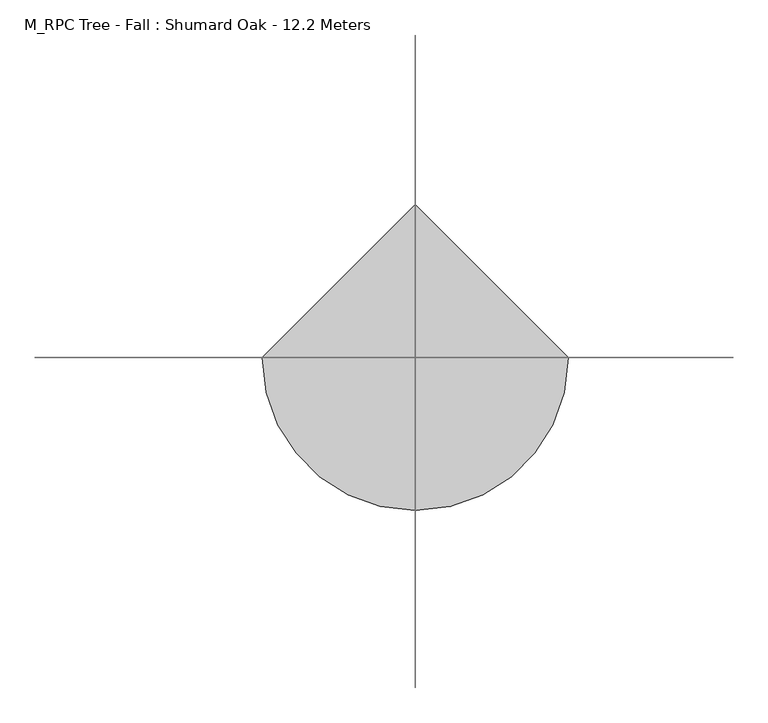
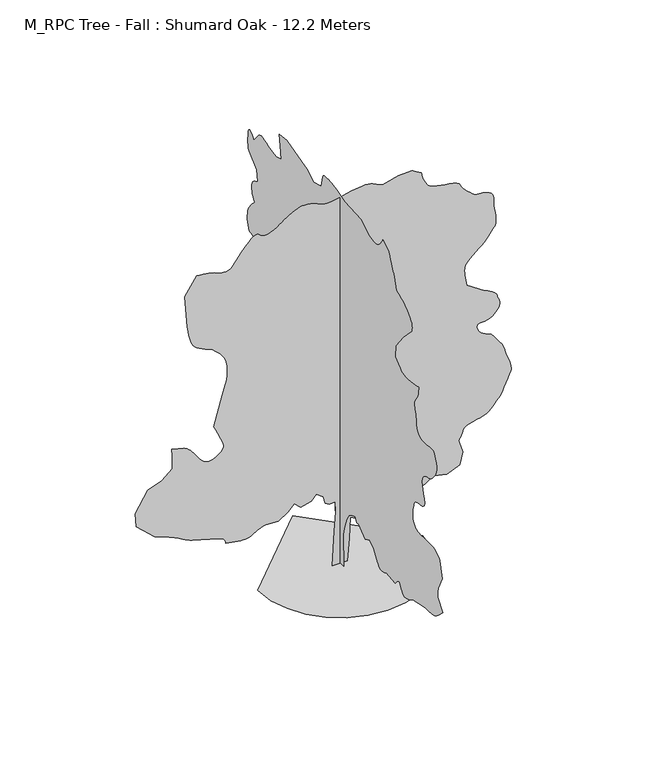
"""IFC4 building model written with IfcOpenShell, lengths in millimetres: geographic element geometry, M_RPC Tree - Fall : Shumard Oak - 12.2 Meters."""

from ifc_helpers import new_model, si_unit, origin, place, context, project, spatial, triangles, source, transform, mapped, element, save


def m_rpc_tree_fall_shumard_oak_12_2_meters_a262d815(model_context):
    return source(origin(), model_context, "Body", "Tessellation", [
        triangles([(-0.0022625, 219.6430976, 0.0114771), (-0.0022625, -202.2794772, 0.0114771), (-0.0022625, -165.5900743, 1045.6450413), (-0.0022625, -238.9678628, 1357.501878), (-0.0022625, -349.0363624, 1651.0131775), (-0.0022625, -477.4462206, 1852.8008606), (-0.0022625, -624.2017977, 1944.5243317), (-0.0022625, -807.646269, 2017.9021202), (-0.0022625, -881.0241302, 1852.8008606), (-0.0022625, -1009.4364956, 1889.4897549), (-0.0022625, -1156.1920727, 1742.7340324), (-0.0022625, -1357.9797558, 1614.3242832), (-0.0022625, -1596.4563332, 1724.390966), (-0.0022625, -1816.5896988, 1577.6353889), (-0.0022625, -1963.347892, 1320.8129837), (-0.0022625, -1998.8599686, 1270.1093925), (-0.0022625, -2035.172723, 1221.8152473), (-0.0022625, -2073.0917747, 1178.3350525), (-0.0022625, -2113.4178017, 1142.073167), (-0.0022625, -2156.9513363, 1115.4391096), (-0.0022625, -2204.4982887, 1100.8397827), (-0.0022625, -2256.8565754, 1100.6771473), (-0.0022625, -2307.0772018, 1109.6110497), (-0.0022625, -2348.6333862, 1120.4664917), (-0.0022625, -2382.9686451, 1132.928231), (-0.0022625, -2411.5294018, 1146.673613), (-0.0022625, -2435.7565567, 1161.3821629), (-0.0022625, -2457.0962425, 1176.7312986), (-0.0022625, -2476.9897957, 1192.4006184), (-0.0022625, -2953.9455666, 1137.368585), (-0.0022625, -3000.966243, 1191.6508095), (-0.0022625, -3046.9957008, 1241.4419563), (-0.0022625, -3091.1191704, 1282.250948), (-0.0022625, -3132.3701408, 1309.5814018), (-0.0022625, -3169.7582657, 1318.9398422), (-0.0022625, -3202.3167435, 1305.8375896), (-0.0022625, -3229.1060966, 1265.7784069), (-0.0022625, -3256.0221863, 1208.176763), (-0.0022625, -3289.3434082, 1148.6509632), (-0.0022625, -3328.7392593, 1092.0151033), (-0.0022625, -3373.9553947, 1043.0779741), (-0.0022625, -3424.5851532, 1006.655924), (-0.0022625, -3480.3747711, 987.5629761), (-0.0022625, -3540.9678749, 990.6103918), (-0.0022625, -3601.7135857, 1008.4757984), (-0.0022625, -3658.6214493, 1030.1891533), (-0.0022625, -3712.3268921, 1055.1127047), (-0.0022625, -3763.4650497, 1082.6007797), (-0.0022625, -3812.6716393, 1112.0180248), (-0.0022625, -3860.5820869, 1142.7162237), (-0.0022625, -3907.8568176, 1174.0574793), (-0.0022625, -4568.2572052, 1302.4673012), (-0.0022625, -4650.6324097, 1302.6274658), (-0.0022625, -4731.8637886, 1303.7507984), (-0.0022625, -4810.8586761, 1306.8009029), (-0.0022625, -4886.4732468, 1312.7355698), (-0.0022625, -4957.6142532, 1322.5236351), (-0.0022625, -5023.1381607, 1337.1228893), (-0.0022625, -5081.9014343, 1357.501878), (-0.0022625, -5138.5299545, 1386.9699921), (-0.0022625, -5198.0553909, 1427.0265587), (-0.0022625, -5259.9957962, 1475.9103481), (-0.0022625, -5323.8680603, 1531.8524277), (-0.0022625, -5389.1634933, 1593.0911316), (-0.0022625, -5455.4245651, 1657.8578178), (-0.0022625, -5522.1681656, 1724.390966), (-0.0022625, -5265.3588409, 2017.9021202), (-0.0022625, -5257.7087265, 2072.8807411), (-0.0022625, -5251.3288834, 2127.5393234), (-0.0022625, -5247.5419052, 2181.5572472), (-0.0022625, -5247.5924835, 2234.6118576), (-0.0022625, -5252.7776321, 2286.3829708), (-0.0022625, -5264.3932022, 2336.5504028), (-0.0022625, -5283.6844666, 2384.7910629), (-0.0022625, -5485.4924973, 2806.7071701), (-0.0022625, -5357.0619644, 3320.3516899), (-0.0022625, -5347.0224609, 3334.5342545), (-0.0022625, -5317.0562668, 3370.8544212), (-0.0022625, -5267.544754, 3419.9848526), (-0.0022625, -5198.7675568, 3472.673497), (-0.0022625, -5111.054306, 3519.5671463), (-0.0022625, -5004.7369583, 3551.3887505), (-0.0022625, -4880.1189835, 3558.8359703), (-0.0022625, -4741.2681564, 3553.0662643), (-0.0022625, -4598.2742683, 3550.8041931), (-0.0022625, -4460.38908, 3551.1346962), (-0.0022625, -4336.9405106, 3553.0662643), (-0.0022625, -4237.2564789, 3555.6332588), (-0.0022625, -4170.614035, 3557.8700409), (-0.0022625, -4146.341098, 3558.8359703), (-0.0022625, -4132.1076645, 3568.5196815), (-0.0022625, -4095.4317055, 3595.8424324), (-0.0022625, -4045.2591866, 3638.2628082), (-0.0022625, -3990.588105, 3693.1882347), (-0.0022625, -3940.4411659, 3758.0514267), (-0.0022625, -3903.7393364, 3830.3106789), (-0.0022625, -3889.5061935, 3907.3739983), (-0.0022625, -3892.2002151, 3984.3864487), (-0.0022625, -3899.6727242, 4058.5266907), (-0.0022625, -3911.1609764, 4130.2522545), (-0.0022625, -3925.8772293, 4200.0465408), (-0.0022625, -3943.0081604, 4268.3917877), (-0.0022625, -3961.7148674, 4335.7711052), (-0.0022625, -3981.2346062, 4402.667894), (-0.0022625, -3997.2725807, 4422.2640816), (-0.0022625, -4015.2421234, 4441.35187), (-0.0022625, -4037.0750931, 4459.4740196), (-0.0022625, -4064.677478, 4476.1727097), (-0.0022625, -4099.9558479, 4490.9142517), (-0.0022625, -4144.8923492, 4503.2922752), (-0.0022625, -4201.3679718, 4512.7472214), (-0.0022625, -4269.6626404, 4518.5166367), (-0.0022625, -4343.4215103, 4525.252272), (-0.0022625, -4414.6136765, 4540.6545296), (-0.0022625, -4475.2067802, 4572.4255554), (-0.0022625, -4517.1952057, 4628.2657516), (-0.0022625, -4532.5213051, 4715.8769737), (-0.0022625, -4513.2300407, 4842.9346252), (-0.0022625, -4473.7071625, 4986.5892288), (-0.0022625, -4437.3869957, 5118.3747894), (-0.0022625, -4409.7337418, 5237.654718), (-0.0022625, -4396.2118927, 5343.7435913), (-0.0022625, -4402.2612328, 5436.0571426), (-0.0022625, -4433.3200928, 5513.9332031), (-0.0022625, -4494.8794167, 5576.7125107), (-0.0022625, -4570.3413803, 5620.6830826), (-0.0022625, -4640.3641411, 5647.6500412), (-0.0022625, -4706.1929718, 5665.2896622), (-0.0022625, -4769.1501755, 5681.3276367), (-0.0022625, -4830.4804436, 5703.465239), (-0.0022625, -4891.5054977, 5739.4299042), (-0.0022625, -4953.4970627, 5796.846167), (-0.0022625, -5016.6571609, 5869.9184509), (-0.0022625, -5076.9197617, 5947.7950928), (-0.0022625, -5129.1764557, 6030.7807251), (-0.0022625, -5168.2670929, 6119.2555573), (-0.0022625, -5189.0838455, 6213.4753876), (-0.0022625, -5186.4654007, 6313.8198441), (-0.0022625, -5155.2795135, 6420.5697235), (-0.0022625, -5117.6376251, 6521.5501877), (-0.0022625, -5092.1699936, 6603.8998123), (-0.0022625, -5068.6342209, 6667.0093323), (-0.0022625, -5036.7617477, 6710.2177414), (-0.0022625, -4986.2845963, 6732.9146118), (-0.0022625, -4906.908046, 6734.4145203), (-0.0022625, -4788.3905708, 6714.0808777), (-0.0022625, -4647.7857811, 6691.613063), (-0.0022625, -4512.6454834, 6687.1139191), (-0.0022625, -4388.3835915, 6700.6101883), (-0.0022625, -4280.5154663, 6732.0507111), (-0.0022625, -4194.4803108, 6781.4604858), (-0.0022625, -4135.6914574, 6848.8656738), (-0.0022625, -4109.6395592, 6934.214534), (-0.0022625, -4100.7183014, 7025.3583893), (-0.0022625, -4089.8654755, 7110.7072495), (-0.0022625, -4077.385714, 7191.2529144), (-0.0022625, -4063.6609703, 7267.9348618), (-0.0022625, -4048.9447174, 7341.7448914), (-0.0022625, -4033.5930382, 7413.6230621), (-0.0022625, -4017.9364357, 7484.5350128), (-0.0022625, -4002.6864944, 7535.6737518), (-0.0022625, -3990.3337601, 7586.9642258), (-0.0022625, -3983.7510223, 7638.5854935), (-0.0022625, -3985.8351974, 7690.6642914), (-0.0022625, -3999.483783, 7743.4035141), (-0.0022625, -4027.5436981, 7796.9310608), (-0.0022625, -4072.9633095, 7851.4242462), (-0.0022625, -4121.5091835, 7918.2951645), (-0.0022625, -4158.2107224, 8002.1446976), (-0.0022625, -4184.6184128, 8093.0600784), (-0.0022625, -4202.3847702, 8181.1029602), (-0.0022625, -4213.0852798, 8256.2855804), (-0.0022625, -4218.3210068, 8308.7201706), (-0.0022625, -4219.7188866, 8328.392807), (-0.0022625, -4192.65019, 8322.3431763), (-0.0022625, -4120.0348549, 8306.9917877), (-0.0022625, -4014.6575661, 8286.5058289), (-0.0022625, -3889.4044556, 8265.0798111), (-0.0022625, -3757.0854973, 8246.830925), (-0.0022625, -3630.5615341, 8235.9775177), (-0.0022625, -3522.6172508, 8236.6641037), (-0.0022625, -3431.498394, 8252.5491806), (-0.0022625, -3346.123954, 8282.871167), (-0.0022625, -3265.5788704, 8325.2406738), (-0.0022625, -3188.8969231, 8377.2177338), (-0.0022625, -3115.0868935, 8436.4385376), (-0.0022625, -3043.2087227, 8500.4375381), (-0.0022625, -2972.2964813, 8566.876506), (-0.0022625, -2990.6471054, 8952.1163635), (-0.0022625, -3394.2122978, 9465.761174), (-0.0022625, -3852.8299438, 9942.7035736), (-0.0022625, -3859.9975296, 10001.8488007), (-0.0022625, -3862.9964745, 10062.1369812), (-0.0022625, -3857.6337204, 10124.6622345), (-0.0022625, -3839.7659157, 10190.5419342), (-0.0022625, -3805.2247101, 10260.9201965), (-0.0022625, -3749.8164642, 10336.9155579), (-0.0022625, -3669.3728279, 10419.6721344), (-0.0022625, -3575.0262611, 10499.1754211), (-0.0022625, -3480.7049835, 10566.1992371), (-0.0022625, -3386.3587074, 10622.777179), (-0.0022625, -3292.0121407, 10671.0172577), (-0.0022625, -3197.6655739, 10713.0053925), (-0.0022625, -3103.3190071, 10750.825177), (-0.0022625, -3008.9724403, 10786.535788), (-0.0022625, -2981.4465042, 10880.6288818), (-0.0022625, -2953.7423813, 10973.0941681), (-0.0022625, -2925.7077553, 11062.3573242), (-0.0022625, -2897.1903099, 11146.8172852), (-0.0022625, -2868.0627274, 11224.8462433), (-0.0022625, -2838.0965332, 11294.8431335), (-0.0022625, -2807.1899895, 11355.2324707), (-0.0022625, -2772.9028381, 11421.0621735), (-0.0022625, -2735.1083427, 11502.2932617), (-0.0022625, -2696.9580551, 11589.6507202), (-0.0022625, -2661.7305542, 11673.779306), (-0.0022625, -2632.5776825, 11745.3784241), (-0.0022625, -2612.7274406, 11795.1695709), (-0.0022625, -2605.4075386, 11813.8509888), (-0.0022625, -2293.5479404, 11997.2828156), (-0.0022625, -2277.555748, 11965.6638153), (-0.0022625, -2259.9598743, 11933.1053375), (-0.0022625, -2239.1538769, 11898.6155823), (-0.0022625, -2213.5363998, 11861.2271667), (-0.0022625, -2181.5012913, 11819.9761963), (-0.0022625, -2141.4421085, 11773.9464478), (-0.0022625, -2091.7577866, 11722.1217041), (-0.0022625, -2031.9117302, 11677.2360718), (-0.0022625, -1963.4012318, 11650.6760651), (-0.0022625, -1887.6698078, 11639.3151306), (-0.0022625, -1806.1612656, 11640.1790314), (-0.0022625, -1720.3217377, 11650.1935364), (-0.0022625, -1631.594886, 11666.2820892), (-0.0022625, -1541.4242271, 11685.4204559), (-0.0022625, -1137.8463902, 11960.5804047), (-0.0022625, -257.3128368, 12015.6328583), (-0.0022625, -143.5556361, 12046.9216461), (-0.0022625, -31.2426242, 12077.2430511), (-0.0022625, 78.1820465, 12105.6331787), (-0.0022625, 183.2749686, 12131.1513885), (-0.0022625, 282.5921986, 12152.8070435), (-0.0022625, 374.6893387, 12169.6583405), (-0.0022625, 458.1194206, 12180.7390594), (-0.0022625, 540.3752283, 12189.1780792), (-0.0022625, 626.4842165, 12196.675296), (-0.0022625, 711.3070913, 12199.9797455), (-0.0022625, 789.7123346, 12195.9137146), (-0.0022625, 856.5631233, 12181.2739105), (-0.0022625, 906.7304827, 12152.8070435), (-0.0022625, 935.0776623, 12107.3365631), (-0.0022625, 1026.7985899, 11740.4729095), (-0.0022625, 1430.3764996, 11630.3935822), (-0.0022625, 1797.2654423, 11850.5266571), (-0.0022625, 2255.8780014, 11960.5804047), (-0.0022625, 2861.2512245, 12144.0378113), (-0.0022625, 3264.8164169, 12089.0109375), (-0.0022625, 3228.1401672, 11740.4729095), (-0.0022625, 3154.7623787, 11336.882428), (-0.0022625, 3448.2735329, 11245.1531433), (-0.0022625, 3741.784687, 11300.1811798), (-0.0022625, 3855.2699112, 11342.8297394), (-0.0022625, 3965.7050308, 11381.7424805), (-0.0022625, 4070.0405228, 11413.310321), (-0.0022625, 4165.2509903, 11433.7962799), (-0.0022625, 4248.2619118, 11439.5145355), (-0.0022625, 4316.0226013, 11426.7804291), (-0.0022625, 4365.4832451, 11391.9093018), (-0.0022625, 4640.6437752, 11061.7213165), (-0.0022625, 4703.1684471, 11134.820343), (-0.0022625, 4763.4566277, 11198.46297), (-0.0022625, 4819.2209564, 11243.1707062), (-0.0022625, 4868.274939, 11259.4883148), (-0.0022625, 4908.3317963, 11237.9349792), (-0.0022625, 4937.1538742, 11169.0566254), (-0.0022625, 4952.5058441, 11043.3712738), (-0.0022625, 4957.156723, 10903.7832825), (-0.0022625, 4956.038768, 10795.9654449), (-0.0022625, 4950.1164551, 10714.6064575), (-0.0022625, 4940.305426, 10654.4461761), (-0.0022625, 4927.6480591, 10610.169809), (-0.0022625, 4913.0338348, 10576.467215), (-0.0022625, 4897.478389, 10548.0770874), (-0.0022625, 4475.5625725, 10199.5134796), (-0.0022625, 4438.8610336, 9814.2997833), (-0.0022625, 4497.5481491, 9790.3826385), (-0.0022625, 4554.4304329, 9764.5586334), (-0.0022625, 4607.8053726, 9734.8726547), (-0.0022625, 4655.8937164, 9699.416098), (-0.0022625, 4696.9159218, 9656.2588486), (-0.0022625, 4729.118898, 9603.4684662), (-0.0022625, 4750.7231026, 9539.1136734), (-0.0022625, 4758.958065, 9468.3790375), (-0.0022625, 4753.7223381, 9397.6194031), (-0.0022625, 4737.2521225, 9326.8591873), (-0.0022625, 4711.7847816, 9256.0995529), (-0.0022625, 4679.5818054, 9185.3393372), (-0.0022625, 4642.9058464, 9114.5797028), (-0.0022625, 4603.9675255, 9043.819487), (-0.0022625, 4662.6799301, 8984.827739), (-0.0022625, 4719.9688751, 8925.6830933), (-0.0022625, 4774.3606133, 8866.2082352), (-0.0022625, 4824.4313942, 8806.250267), (-0.0022625, 4868.7068893, 8745.6574539), (-0.0022625, 4905.7645111, 8684.2763168), (-0.0022625, 4934.1546387, 8621.9039612), (-0.0022625, 4954.5388596, 8561.1582504), (-0.0022625, 4969.1536652, 8504.2500961), (-0.0022625, 4978.9391144, 8450.5446533), (-0.0022625, 4984.8608459, 8399.4064957), (-0.0022625, 4987.9112411, 8350.2001968), (-0.0022625, 4989.0291962, 8302.2897491), (-0.0022625, 4989.2070923, 8255.0147278), (-0.0022625, 4879.1277649, 7943.1529495), (-0.0022625, 4828.0657654, 7934.9685654), (-0.0022625, 4777.130793, 7924.8784836), (-0.0022625, 4726.5519035, 7910.8991043), (-0.0022625, 4676.4302536, 7891.1758896), (-0.0022625, 4626.9696098, 7863.7258209), (-0.0022625, 4578.2967087, 7826.6681992), (-0.0022625, 4530.5897369, 7778.046167), (-0.0022625, 4487.1525627, 7720.3508514), (-0.0022625, 4450.476313, 7657.8255981), (-0.0022625, 4419.3918732, 7591.3104721), (-0.0022625, 4392.8059959, 7521.5670547), (-0.0022625, 4369.6007263, 7449.4092499), (-0.0022625, 4348.6319481, 7375.6503799), (-0.0022625, 4328.8069954, 7301.103186), (-0.0022625, 4285.8529312, 7242.111438), (-0.0022625, 4244.6781189, 7182.9667923), (-0.0022625, 4207.0106506, 7123.4919342), (-0.0022625, 4174.6553581, 7063.5339661), (-0.0022625, 4149.3656227, 7002.941153), (-0.0022625, 4132.8956978, 6941.534436), (-0.0022625, 4126.9989647, 6879.1876602), (-0.0022625, 4145.3498795, 6383.8684753), (-0.0022625, 4188.3039436, 6379.5472275), (-0.0022625, 4229.478756, 6372.8121735), (-0.0022625, 4267.1462242, 6361.2477631), (-0.0022625, 4299.5018074, 6342.4901871), (-0.0022625, 4324.7912521, 6314.0744797), (-0.0022625, 4341.2611771, 6273.6618301), (-0.0022625, 4347.1323303, 6218.7872726), (-0.0022625, 4345.5312653, 6155.3475403), (-0.0022625, 4341.0579918, 6090.9671677), (-0.0022625, 4334.1444603, 6025.7734726), (-0.0022625, 4325.3249405, 5959.9187714), (-0.0022625, 4315.0566719, 5893.6071213), (-0.0022625, 4303.8224739, 5826.9646774), (-0.0022625, 4292.1054565, 5760.1699173), (-0.0022625, 4273.7545418, 5393.2806839), (-0.0022625, 4622.3181496, 5411.631308), (-0.0022625, 5007.5327179, 5485.0093872), (-0.0022625, 5089.5265503, 5457.2541046), (-0.0022625, 5168.1403564, 5428.0506546), (-0.0022625, 5240.0441071, 5395.949707), (-0.0022625, 5301.8060349, 5359.5275116), (-0.0022625, 5350.0978546, 5317.3359009), (-0.0022625, 5381.5383774, 5267.9261261), (-0.0022625, 5392.7725754, 5209.8232773), (-0.0022625, 5389.5698639, 5136.2423035), (-0.0022625, 5380.5721573, 5043.3956451), (-0.0022625, 5366.7968353, 4934.5104309), (-0.0022625, 5349.1322159, 4812.790535), (-0.0022625, 5328.5956787, 4681.4372154), (-0.0022625, 5306.1272827, 4543.6537651), (-0.0022625, 5282.7182465, 4402.667894), (-0.0022625, 5117.6120453, 3962.400872), (-0.0022625, 5027.4338287, 3911.8219826), (-0.0022625, 4938.704361, 3864.2673271), (-0.0022625, 4852.8723907, 3822.8128807), (-0.0022625, 4771.3613777, 3790.5084572), (-0.0022625, 4695.6453598, 3770.4038704), (-0.0022625, 4627.1219261, 3765.5492249), (-0.0022625, 4567.2659866, 3778.9693359), (-0.0022625, 4053.6211761, 3999.1027016), (-0.0022625, 3539.9766563, 3833.9962097), (-0.0022625, 3173.0877136, 3577.1865944), (-0.0022625, 2806.1987709, 3026.8405357), (-0.0022625, 2770.6916359, 2972.1438744), (-0.0022625, 2734.3967583, 2919.353492), (-0.0022625, 2696.4752357, 2870.4012474), (-0.0022625, 2656.139035, 2827.2437073), (-0.0022625, 2612.6004135, 2791.7874413), (-0.0022625, 2565.0713379, 2765.9643082), (-0.0022625, 2512.700116, 2751.6800056), (-0.0022625, 2460.4463287, 2746.9270981), (-0.0022625, 2411.4048454, 2747.2828903), (-0.0022625, 2362.0407074, 2751.1971863), (-0.0022625, 2308.8259323, 2757.0174706), (-0.0022625, 2248.2300671, 2763.1682579), (-0.0022625, 2176.7229492, 2768.0484833), (-0.0022625, 2090.7765965, 2770.0309204), (-0.0022625, 1998.5727768, 2763.0668106), (-0.0022625, 1910.2194489, 2743.5976501), (-0.0022625, 1825.0763901, 2713.7076141), (-0.0022625, 1742.5003258, 2675.4555885), (-0.0022625, 1661.8482719, 2630.9766174), (-0.0022625, 1582.4797153, 2582.3037163), (-0.0022625, 1503.7542881, 2531.54664), (-0.0022625, 1393.6876053, 2219.6898033), (-0.0022625, 1081.8332394, 1871.1465431), (-0.0022625, 1038.7799807, 1824.5095642), (-0.0022625, 988.9862904, 1778.8358986), (-0.0022625, 933.5780445, 1733.9627655), (-0.0022625, 873.678721, 1689.7327618), (-0.0022625, 810.4091091, 1645.9857227), (-0.0022625, 744.8926867, 1602.5563969), (-0.0022625, 678.2553297, 1559.2895611), (-0.0022625, 568.1886469, 1944.5243317), (-0.0022625, 384.7416321, 2201.3465916), (-0.0022625, 311.3663507, 2036.245332), (-0.0022625, 256.3317375, 1779.4229267), (-0.0022625, 237.9877991, 1320.8129837), (-0.0022625, 201.2983961, 678.7560259), (227.2985896, 0.0005818, 0.0290512), (-249.6563274, 0.0005818, 0.0290512), (-176.2792837, 0.0005163, 1100.6948788), (-139.5901351, 0.0004777, 1742.7519093), (-157.9345822, 0.0004581, 2072.9519577), (-341.3808703, 0.0004592, 2054.608746), (-469.7907286, 0.000455, 2127.9865345), (-524.8227983, 0.0004406, 2366.4631119), (-744.9587437, 0.0004319, 2513.218689), (-891.7143208, 0.0004417, 2348.1174294), (-1221.9118984, 0.0004473, 2256.3964291), (-1423.7020523, 0.0004364, 2439.8409004), (-1625.4897354, 0.0004483, 2238.0507465), (-1919.0008896, 0.0004592, 2054.608746), (-2359.270237, 0.0004581, 2072.9519577), (-2579.4062187, 0.0004637, 1981.2284866), (-2626.6812401, 0.0004658, 1946.0925499), (-2674.5913971, 0.0004679, 1912.3976589), (-2723.7979866, 0.0004697, 1881.5927078), (-2774.9361443, 0.0004711, 1855.1187424), (-2828.6415871, 0.0004725, 1834.4220406), (-2885.5241615, 0.0004732, 1820.9436481), (-2946.2951614, 0.0004735, 1816.1296978), (-3014.004982, 0.0004735, 1818.2698288), (-3090.3820061, 0.0004732, 1824.2579807), (-3173.9771942, 0.0004725, 1833.4587273), (-3263.3420883, 0.0004718, 1845.2241428), (-3357.0279396, 0.0004711, 1858.9160397), (-3453.6362869, 0.00047, 1873.8915791), (-3551.6683846, 0.0004693, 1889.5074863), (-3556.192527, 0.0004669, 1928.7100353), (-3564.4527786, 0.0004644, 1967.2696003), (-3580.0588028, 0.0004623, 2004.5482841), (-3606.7461273, 0.0004602, 2039.9001961), (-3648.2005737, 0.0004581, 2072.6851135), (-3708.0823837, 0.0004564, 2102.2599072), (-3790.1270851, 0.000455, 2127.9865345), (-4597.2827591, 0.0004406, 2366.4631119), (-4663.1883293, 0.0004396, 2387.3759342), (-4733.5668823, 0.0004378, 2416.9507278), (-4806.1822174, 0.0004357, 2452.6229691), (-4878.822551, 0.0004333, 2491.825518), (-4949.2013947, 0.0004308, 2531.9913803), (-5015.1066742, 0.0004287, 2570.5611191), (-5074.2513199, 0.0004266, 2604.9500084), (-5137.8433685, 0.0004245, 2637.9915962), (-5216.8385468, 0.0004224, 2673.9306816), (-5308.668988, 0.00042, 2712.2844452), (-5410.7674072, 0.0004179, 2752.5441971), (-5520.5671005, 0.0004154, 2794.2782776), (-5635.5013641, 0.0004126, 2836.9527077), (-5753.0023315, 0.0004101, 2880.1102478), (-6321.6740158, 0.0003783, 3412.1056824), (-6358.3502655, 0.000352, 3852.3724136), (-5973.1354065, 0.0003149, 4476.0709717), (-5532.8686752, 0.0003051, 4641.1774635), (-5202.6562729, 0.0002886, 4916.3377029), (-5202.6562729, 0.0002637, 5338.2538101), (-5221.006897, 0.0002504, 5558.3868851), (-4835.7670395, 0.000256, 5466.6837616), (-4792.4063141, 0.0002578, 5438.7000046), (-4748.2066864, 0.0002595, 5407.9972275), (-4702.4315735, 0.0002616, 5371.8546661), (-4654.2414917, 0.0002641, 5327.5027222), (-4602.8489891, 0.0002676, 5272.2723724), (-4547.4407433, 0.0002718, 5203.3928558), (-4487.2290115, 0.0002767, 5118.1201538), (-4426.2036667, 0.000282, 5028.5523651), (-4367.4148132, 0.0002869, 4949.5571869), (-4308.6515396, 0.0002907, 4882.7624268), (-4247.6264854, 0.0002939, 4829.7432793), (-4182.1022873, 0.0002963, 4792.1522598), (-4109.8427444, 0.0002974, 4771.564563), (-4028.6113655, 0.0002974, 4769.5821259), (-3939.7801598, 0.0002963, 4789.9154778), (-3850.3138184, 0.0002939, 4831.0902901), (-3766.2863892, 0.0002904, 4887.032515), (-3693.823661, 0.0002865, 4951.641362), (-3638.9999725, 0.0002827, 5018.8174942), (-3607.915242, 0.0002788, 5082.4607025), (-3606.6952583, 0.0002756, 5136.4713593), (-3628.2994629, 0.0002721, 5194.8788406), (-3660.5024391, 0.0002676, 5273.4920654), (-3701.5246445, 0.0002616, 5368.9571686), (-3749.5876991, 0.0002553, 5477.9179596), (-3802.9626389, 0.0002483, 5596.9694138), (-3859.8702118, 0.0002406, 5722.7565033), (-3918.5573273, 0.0002329, 5851.8980392), (-3661.7224228, 0.0001772, 6787.4845367), (-3626.5966599, 0.0001709, 6893.3699341), (-3592.8940659, 0.0001646, 6997.8321625), (-3562.0892601, 0.0001587, 7099.3968933), (-3535.6051208, 0.0001527, 7196.6159592), (-3514.9159767, 0.0001475, 7288.064447), (-3501.4449966, 0.0001422, 7372.2953522), (-3496.6159309, 0.000138, 7447.884343), (-3497.8612038, 0.0001334, 7521.6182144), (-3501.9789757, 0.0001289, 7599.875647), (-3509.6293808, 0.000124, 7680.3701523), (-3521.4478455, 0.0001191, 7760.8646576), (-3538.0703773, 0.0001145, 7839.0970917), (-3560.1574013, 0.00011, 7912.8559616), (-3588.3446342, 0.0001061, 7979.8541977), (-3624.613932, 0.0001023, 8042.2265533), (-3669.5251442, 9.88e-05, 8103.6332703), (-3721.6801003, 9.53e-05, 8164.2266647), (-3779.6047623, 9.14e-05, 8224.1846329), (-3841.8500908, 8.79e-05, 8283.6339111), (-3906.9926262, 8.44e-05, 8342.8035553), (-3973.584201, 8.09e-05, 8401.7958847), (-4079.2667038, 7.85e-05, 8445.1054504), (-4182.2040253, 7.57e-05, 8488.8987076), (-4279.7021439, 7.32e-05, 8533.6826019), (-4369.0414581, 7.04e-05, 8579.8902466), (-4447.4264992, 6.76e-05, 8628.0291687), (-4512.213533, 6.44e-05, 8678.5574799), (-4560.6068001, 6.13e-05, 8731.9832886), (-4598.6809296, 5.71e-05, 8803.226033), (-4633.8828506, 5.15e-05, 8899.8090912), (-4665.5265587, 4.48e-05, 9011.1592712), (-4693.0272057, 3.78e-05, 9126.6778015), (-4715.6990776, 3.12e-05, 9235.7914902), (-4732.931456, 2.59e-05, 9327.8759857), (-4744.0383362, 2.21e-05, 9392.3830948), (-4817.4161247, -3.92e-05, 10419.6721344), (-4450.527182, -7.32e-05, 10988.3444), (-4352.4953751, -7.25e-05, 10976.4241974), (-4255.9123169, -7.18e-05, 10963.6900909), (-4162.2011765, -7.08e-05, 10949.3549194), (-4072.8362823, -6.97e-05, 10932.6303589), (-3989.2410942, -6.86e-05, 10912.6792511), (-3912.8893593, -6.72e-05, 10888.7109467), (-3845.1795387, -6.55e-05, 10859.939447), (-3776.3258926, -6.37e-05, 10832.1330048), (-3698.8306229, -6.27e-05, 10812.6644257), (-3617.497506, -6.2e-05, 10803.1336121), (-3537.1047386, -6.23e-05, 10805.1660461), (-3462.5069664, -6.3e-05, 10820.3651184), (-3398.482386, -6.48e-05, 10850.3063141), (-3349.8603539, -6.76e-05, 10896.6406952), (-3056.3491997, -9.07e-05, 11281.8555542), (-2977.9641586, -9.6e-05, 11371.601239), (-2900.8246811, -0.0001012, 11457.3320526), (-2826.2777779, -0.0001058, 11535.0552155), (-2755.5687218, -0.0001096, 11600.7326019), (-2689.9939453, -0.0001128, 11650.3714325), (-2630.8492996, -0.0001145, 11679.9300934), (-2579.4062187, -0.0001149, 11685.4460358), (-2538.0075829, -0.0001138, 11671.6445526), (-2504.3128372, -0.0001124, 11649.1761566), (-2472.5444275, -0.000111, 11622.8696228), (-2436.9256714, -0.0001096, 11597.5293091), (-2391.6790146, -0.0001082, 11577.9339935), (-2331.0324257, -0.0001079, 11568.9612854), (-2249.2035542, -0.0001082, 11575.3667084), (-2151.4359753, -0.00011, 11603.1975677), (-2051.1038727, -0.0001124, 11649.6086884), (-1954.619791, -0.0001159, 11706.3133667), (-1868.4065941, -0.0001194, 11764.9237427), (-1798.8794426, -0.0001226, 11817.1298584), (-1752.4584389, -0.0001247, 11854.542691), (-1735.5564182, -0.0001257, 11868.8778625), (-1714.8597164, -0.0001264, 11882.1456573), (-1659.8251396, -0.0001285, 11916.5842529), (-1581.0462273, -0.0001313, 11964.1894867), (-1489.1092518, -0.0001345, 12016.9292908), (-1394.6076073, -0.0001373, 12066.7715973), (-1308.1275661, -0.0001398, 12105.7099182), (-1240.2575809, -0.0001408, 12125.7121857), (-1175.8645638, -0.0001412, 12130.1607513), (-1095.7488144, -0.0001412, 12127.5167267), (-1004.4014832, -0.0001405, 12117.5289642), (-906.3136477, -0.0001394, 12099.8126038), (-805.9815451, -0.000138, 12074.090918), (-707.8936369, -0.0001359, 12040.0336945), (-616.5463057, -0.0001334, 11997.3083954), (-519.3684073, -0.0001313, 11962.4361053), (-402.9373964, -0.0001306, 11949.7019989), (-270.4608533, -0.0001306, 11955.4214172), (-125.1499373, -0.000132, 11975.9073761), (29.7882844, -0.0001338, 12007.4496368), (191.1444556, -0.0001362, 12046.386795), (355.7107369, -0.0001387, 12089.0109375), (469.3052567, -0.0001398, 12104.4134857), (580.4953812, -0.0001405, 12117.9091736), (686.8715916, -0.0001412, 12127.5167267), (786.0294926, -0.0001412, 12131.3804443), (875.5569494, -0.0001412, 12127.5167267), (953.0548353, -0.0001401, 12114.0466187), (1016.1109428, -0.0001387, 12089.0109375), (1069.0029179, -0.0001369, 12059.7057495), (1118.0467993, -0.0001355, 12034.2631165), (1163.8806295, -0.0001341, 12011.9981964), (1207.1498634, -0.0001331, 11992.3261414), (1248.4900726, -0.000132, 11974.5597839), (1288.54911, -0.000131, 11958.089859), (1327.9653088, -0.0001299, 11942.2559418), (1804.9209343, -0.0001376, 12070.6853119), (2226.8445992, -0.0001387, 12089.0109375), (2520.3557533, -0.0001289, 11923.9303162), (2524.5799141, -0.0001264, 11880.4934326), (2530.5708275, -0.0001236, 11835.9380127), (2540.0891418, -0.0001208, 11789.14552), (2554.9045166, -0.000118, 11738.9730011), (2576.7883553, -0.0001145, 11684.3274994), (2607.4661339, -0.000111, 11624.0393188), (2648.768264, -0.0001072, 11557.0410828), (2690.2735794, -0.0001033, 11495.6855255), (2724.713047, -0.0001009, 11450.3929413), (2758.5170883, -9.88e-05, 11416.9705627), (2798.0908356, -9.7e-05, 11391.248877), (2849.8644196, -9.6e-05, 11369.0339539), (2920.2432632, -9.46e-05, 11346.2097656), (3015.6572067, -9.28e-05, 11318.5568024), (3133.2599121, -9.14e-05, 11291.9200562), (3260.1649567, -9e-05, 11271.7143127), (3387.7310074, -8.9e-05, 11253.0840546), (3507.2655716, -8.76e-05, 11231.2760834), (3610.1011551, -8.58e-05, 11201.437207), (3687.5964249, -8.34e-05, 11158.7374878), (3731.0841774, -7.99e-05, 11098.4237274), (3763.2362846, -7.57e-05, 11028.1977814), (3810.7909401, -7.15e-05, 10958.9368927), (3871.1552788, -6.72e-05, 10890.4899078), (3941.8134659, -6.34e-05, 10822.6533508), (4020.1729271, -5.92e-05, 10755.3249023), (4103.6410881, -5.53e-05, 10688.3266663), (4189.7018234, -5.11e-05, 10621.4551666), (4310.7357147, -5.04e-05, 10609.0512726), (4426.788224, -4.97e-05, 10592.9627197), (4532.9026772, -4.83e-05, 10569.4781067), (4624.0721123, -4.62e-05, 10534.9371918), (4695.3657257, -4.31e-05, 10485.6285736), (4741.8018448, -3.92e-05, 10417.8675934), (4758.3735077, -3.4e-05, 10327.9440125), (4759.4408844, -2.84e-05, 10234.3090302), (4762.4401199, -2.35e-05, 10156.0510162), (4767.0404205, -1.96e-05, 10090.6538452), (4772.9371536, -1.65e-05, 10035.5258148), (4779.7742363, -1.37e-05, 9988.0728973), (4787.2467453, -1.09e-05, 9945.7789673), (4795.0750465, -8.8e-06, 9906.0279053), (4810.4267258, -3.2e-06, 9812.0115509), (4823.5163338, 2.5e-06, 9719.9020569), (4832.1323776, 7.7e-06, 9631.6556992), (4834.0133675, 1.26e-05, 9549.2037552), (4826.8966507, 1.72e-05, 9474.4280869), (4808.5457359, 2.1e-05, 9409.2855515), (4776.7241318, 2.42e-05, 9355.7074265), (4736.1338768, 2.73e-05, 9304.3146332), (4692.3156212, 3.08e-05, 9245.5263611), (4644.3545952, 3.47e-05, 9180.9680923), (4591.2337097, 3.85e-05, 9112.2414734), (4532.0384857, 4.27e-05, 9040.9475693), (4465.7771233, 4.73e-05, 8968.6880264), (4391.484565, 5.15e-05, 8897.0894897), (4305.2203537, 5.6e-05, 8823.2288818), (4209.0183769, 6.06e-05, 8744.2337036), (4110.8595428, 6.55e-05, 8661.7061829), (4018.8259163, 7.04e-05, 8577.2723831), (3940.8984055, 7.57e-05, 8492.4822098), (3885.1090782, 8.06e-05, 8409.0140488), (3859.4891304, 8.55e-05, 8328.4178055), (3855.3716492, 9e-05, 8248.7116241), (3858.0148018, 9.49e-05, 8167.0985825), (3866.2497643, 9.98e-05, 8083.8844757), (3878.9582909, 0.0001051, 7999.3745178), (3895.0724236, 0.00011, 7913.9239197), (3913.3977585, 0.0001152, 7827.8123154), (3932.8669189, 0.0001205, 7741.3954971), (4483.2129776, 0.0001422, 7374.5068451), (4504.5375481, 0.0001429, 7364.9754501), (4559.5900017, 0.0001443, 7338.7706543), (4634.8232002, 0.0001468, 7299.400383), (4716.8173233, 0.0001496, 7250.4225586), (4792.075811, 0.0001531, 7195.3195267), (4847.1029755, 0.0001562, 7137.6747894), (4868.4528351, 0.0001597, 7080.9956909), (4879.890509, 0.0001629, 7027.4425644), (4906.0947235, 0.000166, 6973.9150177), (4934.8662231, 0.0001695, 6915.8889084), (4954.0051712, 0.0001737, 6848.8656738), (4951.3367294, 0.0001783, 6768.3711685), (4914.6604797, 0.0001842, 6669.9324097), (4831.7512962, 0.0001916, 6549.0002563), (4717.4018806, 0.0001975, 6446.0879333), (4599.8500443, 0.0002007, 6392.9417587), (4487.1272736, 0.0002021, 6371.8715332), (4387.2144768, 0.0002024, 6365.2376358), (4308.1687202, 0.0002031, 6355.4016083), (4257.996492, 0.0002049, 6324.6982498), (4244.7289879, 0.0002091, 6255.4891022), (4263.8167763, 0.000214, 6169.1740219), (4303.1361786, 0.0002182, 6097.2958511), (4359.2815887, 0.0002221, 6037.439621), (4428.9232681, 0.0002249, 5987.2165237), (4508.6806091, 0.0002273, 5944.2115906), (4595.1480057, 0.0002298, 5906.0360138), (4684.9957191, 0.0002319, 5870.2492447), (4774.7925636, 0.0002385, 5756.6619919), (4860.9041679, 0.0002452, 5645.4647095), (4939.6194214, 0.0002515, 5539.0962021), (5007.2786636, 0.0002574, 5439.9458588), (5060.1702026, 0.000263, 5350.4030685), (5094.6099609, 0.0002676, 5272.9077988), (5106.9115356, 0.0002711, 5209.8488571), (5121.9077133, 0.0002756, 5134.4377625), (5159.3461258, 0.0002823, 5026.6205063), (5207.9937378, 0.0002897, 4898.9021393), (5256.6663483, 0.0002977, 4763.8127106), (5294.1053421, 0.0003054, 4633.8572708), (5309.0753586, 0.0003124, 4521.541452), (5290.3689423, 0.0003173, 4439.394722), (5246.880899, 0.0003219, 4358.2647903), (5196.3525879, 0.0003285, 4248.566835), (5140.6647079, 0.0003362, 4122.169899), (5081.7746979, 0.0003439, 3990.9947662), (5021.6132538, 0.0003513, 3866.8599014), (4962.0878174, 0.0003576, 3761.6605087), (4905.1290848, 0.0003622, 3687.2659218), (4849.898735, 0.0003657, 3628.324752), (4793.3466637, 0.0003695, 3563.9446701), (4734.2531776, 0.0003734, 3497.6071495), (4671.3215538, 0.0003772, 3432.8965645), (4603.2303612, 0.0003807, 3373.3199684), (4528.7343269, 0.0003839, 3322.4102852), (4446.5114388, 0.000386, 3283.6754402), (4349.3438232, 0.0003877, 3254.9545189), (4237.4087952, 0.0003895, 3229.1313858), (4120.6449921, 0.0003909, 3202.3423233), (4009.0404671, 0.0003926, 3170.7239044), (3912.5082779, 0.0003951, 3130.4641525), (3840.9858994, 0.0003982, 3077.6737701), (3804.4619659, 0.0004024, 3008.5152008), (3784.8913582, 0.0004066, 2939.2040245), (3760.1864708, 0.0004098, 2885.2953964), (3734.1851509, 0.0004122, 2841.9852493), (3710.7764053, 0.0004147, 2804.419519), (3693.7472122, 0.0004168, 2767.8450073), (3687.0118675, 0.0004193, 2727.4070686), (3694.4082184, 0.0004221, 2678.3277969), (3804.4619659, 0.0004431, 2329.7742176), (3712.7335533, 0.0004669, 1926.1963806), (3309.1683609, 0.0004767, 1761.0975918), (2905.5778793, 0.0004714, 1852.8185921), (2502.0100708, 0.0004865, 1595.9963322), (2208.4987713, 0.0004767, 1761.0975918), (1786.5752518, 0.0004658, 1944.5395924), (1758.9270847, 0.0004669, 1928.4431911), (1730.4731529, 0.0004679, 1910.0975086), (1700.4153946, 0.0004693, 1887.2606758), (1667.9532772, 0.0004711, 1857.6858822), (1632.2785652, 0.0004732, 1819.1237011), (1592.5955223, 0.0004763, 1769.3325542), (1548.0986744, 0.0004802, 1706.063015), (1501.4616955, 0.000484, 1639.5832066), (1455.7880299, 0.0004876, 1580.8072884), (1410.9175129, 0.0004907, 1528.449147), (1366.6875092, 0.0004935, 1481.2223785), (1322.937854, 0.000496, 1437.8490086), (1279.5109989, 0.0004984, 1397.0426331), (1236.2443085, 0.0005009, 1357.5197548), (1291.2764145, 0.000524, 972.2850569), (1259.6683147, 0.0005247, 960.6798059), (1227.0969017, 0.000525, 950.1954168), (1192.6014055, 0.0005257, 941.9604544), (1155.2186583, 0.0005261, 937.0931643), (1113.9827305, 0.0005261, 936.7195679), (1067.9328524, 0.0005257, 941.9604544), (1016.1109428, 0.000525, 953.9393017), (962.1463589, 0.0005236, 973.9422232), (910.1083288, 0.0005222, 1001.6463461), (859.6741253, 0.0005201, 1035.7681005), (810.5234917, 0.0005177, 1075.0241346), (762.3360987, 0.0005152, 1118.1307331), (714.7917624, 0.0005124, 1163.8043987), (667.5651392, 0.0005096, 1210.7615616), (319.0192992, 0.0004988, 1394.2086491), (282.3329484, 0.000539, 715.4627243), (-2557.3444839, 0.0, 0.0), (-2489.7390175, -585.9752066, 0.0), (-2297.1926308, -1124.0985374, 0.0), (-1995.1237141, -1598.9547272, 0.0), (-1598.9547272, -1995.1237141, 0.0), (-1124.0985374, -2297.19016, 0.0), (-585.9752066, -2489.7390175, 0.0), (0.0001118, -2557.3444839, 0.0), (585.9752066, -2489.7390175, 0.0), (1124.0985374, -2297.1926308, 0.0), (1598.9547272, -1995.1237141, 0.0), (1995.1237141, -1598.9547272, 0.0), (2297.1926308, -1124.0985374, 0.0), (2489.7390175, -585.9752066, 0.0), (2557.3444839, 0.0002235, 0.0), (-0.0003354, 2557.3444839, 0.0)], [[407, 408, 409], [173, 174, 175], [406, 407, 409], [219, 220, 221], [1, 2, 3], [414, 1, 3], [413, 414, 3], [413, 3, 4], [412, 413, 4], [412, 4, 5], [255, 256, 257], [219, 221, 222], [65, 66, 67], [405, 406, 409], [8, 9, 10], [219, 222, 223], [404, 405, 409], [64, 65, 67], [412, 5, 6], [411, 412, 6], [403, 404, 409], [219, 223, 224], [172, 173, 175], [172, 175, 176], [171, 172, 176], [171, 176, 177], [170, 171, 177], [254, 255, 257], [254, 257, 258], [402, 403, 409], [63, 64, 67], [218, 219, 224], [401, 402, 409], [218, 224, 225], [217, 218, 225], [312, 313, 314], [216, 217, 225], [216, 225, 226], [170, 177, 178], [169, 170, 178], [168, 169, 178], [167, 168, 178], [167, 178, 179], [166, 167, 179], [166, 179, 180], [165, 166, 180], [11, 12, 13], [216, 226, 227], [215, 216, 227], [400, 401, 409], [400, 409, 410], [399, 400, 410], [29, 30, 31], [62, 63, 67], [214, 215, 227], [214, 227, 228], [410, 411, 6], [410, 6, 7], [165, 180, 181], [164, 165, 181], [312, 314, 315], [61, 62, 67], [213, 214, 228], [60, 61, 67], [59, 60, 67], [58, 59, 67], [57, 58, 67], [56, 57, 67], [55, 56, 67], [54, 55, 67], [53, 54, 67], [52, 53, 67], [52, 67, 68], [52, 68, 69], [253, 254, 258], [252, 253, 258], [29, 31, 32], [271, 272, 273], [271, 273, 274], [270, 271, 274], [270, 274, 275], [269, 270, 275], [268, 269, 275], [268, 275, 276], [268, 276, 277], [268, 277, 278], [268, 278, 279], [268, 279, 280], [268, 280, 281], [268, 281, 282], [268, 282, 283], [267, 268, 283], [266, 267, 283], [265, 266, 283], [264, 265, 283], [263, 264, 283], [262, 263, 283], [261, 262, 283], [260, 261, 283], [259, 260, 283], [259, 283, 284], [52, 69, 70], [212, 213, 228], [212, 228, 229], [211, 212, 229], [210, 211, 229], [209, 210, 229], [208, 209, 229], [10, 11, 13], [163, 164, 181], [163, 181, 182], [312, 315, 316], [51, 52, 70], [51, 70, 71], [51, 71, 72], [207, 208, 229], [207, 229, 230], [206, 207, 230], [366, 367, 368], [74, 75, 76], [74, 76, 77], [74, 77, 78], [74, 78, 79], [74, 79, 80], [74, 80, 81], [74, 81, 82], [74, 82, 83], [74, 83, 84], [74, 84, 85], [74, 85, 86], [73, 74, 86], [73, 86, 87], [73, 87, 88], [72, 73, 88], [51, 72, 88], [51, 88, 89], [51, 89, 90], [51, 90, 91], [51, 91, 92], [51, 92, 93], [50, 51, 93], [49, 50, 93], [48, 49, 93], [47, 48, 93], [46, 47, 93], [45, 46, 93], [44, 45, 93], [43, 44, 93], [42, 43, 93], [41, 42, 93], [40, 41, 93], [39, 40, 93], [38, 39, 93], [37, 38, 93], [36, 37, 93], [35, 36, 93], [35, 93, 94], [34, 35, 94], [34, 94, 95], [34, 95, 96], [33, 34, 96], [205, 206, 230], [258, 259, 284], [252, 258, 284], [29, 32, 33], [29, 33, 96], [29, 96, 97], [311, 312, 316], [190, 191, 192], [190, 192, 193], [190, 193, 194], [190, 194, 195], [190, 195, 196], [190, 196, 197], [190, 197, 198], [190, 198, 199], [190, 199, 200], [190, 200, 201], [190, 201, 202], [190, 202, 203], [190, 203, 204], [190, 204, 205], [189, 190, 205], [189, 205, 230], [189, 230, 231], [189, 231, 232], [189, 232, 233], [189, 233, 234], [410, 7, 8], [310, 311, 316], [310, 316, 317], [309, 310, 317], [308, 309, 317], [307, 308, 317], [306, 307, 317], [305, 306, 317], [304, 305, 317], [303, 304, 317], [302, 303, 317], [302, 317, 318], [301, 302, 318], [300, 301, 318], [299, 300, 318], [299, 318, 319], [298, 299, 319], [298, 319, 320], [162, 163, 182], [366, 368, 369], [298, 320, 321], [366, 369, 370], [366, 370, 371], [366, 371, 372], [366, 372, 373], [366, 373, 374], [366, 374, 375], [365, 366, 375], [364, 365, 375], [363, 364, 375], [362, 363, 375], [361, 362, 375], [360, 361, 375], [359, 360, 375], [358, 359, 375], [357, 358, 375], [356, 357, 375], [355, 356, 375], [354, 355, 375], [353, 354, 375], [352, 353, 375], [351, 352, 375], [350, 351, 375], [350, 375, 376], [234, 235, 236], [189, 234, 236], [188, 189, 236], [188, 236, 237], [188, 237, 238], [188, 238, 239], [188, 239, 240], [188, 240, 241], [188, 241, 242], [188, 242, 243], [188, 243, 244], [188, 244, 245], [188, 245, 246], [188, 246, 247], [188, 247, 248], [188, 248, 249], [188, 249, 250], [188, 250, 251], [188, 251, 252], [188, 252, 284], [187, 188, 284], [187, 284, 285], [187, 285, 286], [187, 286, 287], [187, 287, 288], [187, 288, 289], [187, 289, 290], [187, 290, 291], [187, 291, 292], [187, 292, 293], [187, 293, 294], [187, 294, 295], [187, 295, 296], [187, 296, 297], [187, 297, 298], [187, 298, 321], [187, 321, 322], [187, 322, 323], [187, 323, 324], [187, 324, 325], [187, 325, 326], [187, 326, 327], [187, 327, 328], [187, 328, 329], [187, 329, 330], [187, 330, 331], [187, 331, 332], [187, 332, 333], [187, 333, 334], [187, 334, 335], [186, 187, 335], [185, 186, 335], [184, 185, 335], [183, 184, 335], [182, 183, 335], [162, 182, 335], [161, 162, 335], [160, 161, 335], [159, 160, 335], [158, 159, 335], [157, 158, 335], [156, 157, 335], [155, 156, 335], [154, 155, 335], [153, 154, 335], [152, 153, 335], [151, 152, 335], [150, 151, 335], [350, 376, 377], [142, 143, 144], [142, 144, 145], [141, 142, 145], [141, 145, 146], [140, 141, 146], [140, 146, 147], [139, 140, 147], [138, 139, 147], [137, 138, 147], [136, 137, 147], [135, 136, 147], [134, 135, 147], [133, 134, 147], [133, 147, 148], [132, 133, 148], [131, 132, 148], [130, 131, 148], [129, 130, 148], [128, 129, 148], [127, 128, 148], [127, 148, 149], [126, 127, 149], [125, 126, 149], [125, 149, 150], [125, 150, 335], [124, 125, 335], [123, 124, 335], [122, 123, 335], [121, 122, 335], [120, 121, 335], [119, 120, 335], [118, 119, 335], [117, 118, 335], [116, 117, 335], [115, 116, 335], [114, 115, 335], [113, 114, 335], [112, 113, 335], [111, 112, 335], [110, 111, 335], [109, 110, 335], [108, 109, 335], [107, 108, 335], [106, 107, 335], [105, 106, 335], [104, 105, 335], [103, 104, 335], [102, 103, 335], [101, 102, 335], [100, 101, 335], [99, 100, 335], [98, 99, 335], [97, 98, 335], [29, 97, 335], [28, 29, 335], [27, 28, 335], [26, 27, 335], [25, 26, 335], [25, 335, 336], [25, 336, 337], [25, 337, 338], [349, 350, 377], [339, 340, 341], [338, 339, 341], [338, 341, 342], [338, 342, 343], [338, 343, 344], [338, 344, 345], [338, 345, 346], [348, 349, 377], [347, 348, 377], [346, 347, 377], [338, 346, 377], [20, 21, 22], [19, 20, 22], [19, 22, 23], [18, 19, 23], [17, 18, 23], [17, 23, 24], [17, 24, 25], [16, 17, 25], [15, 16, 25], [14, 15, 25], [14, 25, 338], [13, 14, 338], [10, 13, 338], [8, 10, 338], [8, 338, 377], [410, 8, 377], [398, 399, 410], [398, 410, 377], [397, 398, 377], [396, 397, 377], [395, 396, 377], [394, 395, 377], [393, 394, 377], [393, 377, 378], [392, 393, 378], [391, 392, 378], [390, 391, 378], [389, 390, 378], [389, 378, 379], [389, 379, 380], [388, 389, 380], [388, 380, 381], [387, 388, 381], [387, 381, 382], [386, 387, 382], [386, 382, 383], [385, 386, 383], [384, 385, 383], [472, 473, 474], [415, 416, 417], [793, 415, 417], [792, 793, 417], [792, 417, 418], [776, 777, 778], [776, 778, 779], [776, 779, 780], [776, 780, 781], [776, 781, 782], [776, 782, 783], [776, 783, 784], [776, 784, 785], [776, 785, 786], [776, 786, 787], [776, 787, 788], [776, 788, 789], [443, 444, 445], [471, 472, 474], [471, 474, 475], [471, 475, 476], [471, 476, 477], [471, 477, 478], [471, 478, 479], [471, 479, 480], [471, 480, 481], [471, 481, 482], [776, 789, 790], [776, 790, 791], [539, 540, 541], [759, 760, 761], [471, 482, 483], [424, 425, 426], [423, 424, 426], [539, 541, 542], [613, 614, 615], [756, 757, 758], [756, 758, 759], [755, 756, 759], [539, 542, 543], [538, 539, 543], [538, 543, 544], [538, 544, 545], [538, 545, 546], [538, 546, 547], [538, 547, 548], [538, 548, 549], [538, 549, 550], [754, 755, 759], [471, 483, 484], [538, 550, 551], [537, 538, 551], [443, 445, 446], [792, 418, 419], [536, 537, 551], [535, 536, 551], [534, 535, 551], [533, 534, 551], [532, 533, 551], [531, 532, 551], [530, 531, 551], [529, 530, 551], [528, 529, 551], [527, 528, 551], [526, 527, 551], [525, 526, 551], [524, 525, 551], [524, 551, 552], [523, 524, 552], [522, 523, 552], [522, 552, 553], [521, 522, 553], [520, 521, 553], [519, 520, 553], [613, 615, 616], [420, 421, 422], [419, 420, 422], [612, 613, 616], [612, 616, 617], [612, 617, 618], [612, 618, 619], [776, 791, 792], [776, 792, 419], [775, 776, 419], [774, 775, 419], [773, 774, 419], [772, 773, 419], [771, 772, 419], [770, 771, 419], [769, 770, 419], [768, 769, 419], [767, 768, 419], [766, 767, 419], [765, 766, 419], [764, 765, 419], [466, 467, 468], [466, 468, 469], [466, 469, 470], [465, 466, 470], [464, 465, 470], [463, 464, 470], [462, 463, 470], [461, 462, 470], [461, 470, 471], [461, 471, 484], [461, 484, 485], [461, 485, 486], [460, 461, 486], [459, 460, 486], [459, 486, 487], [458, 459, 487], [457, 458, 487], [456, 457, 487], [455, 456, 487], [454, 455, 487], [453, 454, 487], [452, 453, 487], [451, 452, 487], [451, 487, 488], [451, 488, 489], [450, 451, 489], [450, 489, 490], [449, 450, 490], [449, 490, 491], [449, 491, 492], [448, 449, 492], [518, 519, 553], [518, 553, 554], [611, 612, 619], [611, 619, 620], [611, 620, 621], [448, 492, 493], [754, 759, 761], [754, 761, 762], [753, 754, 762], [752, 753, 762], [501, 502, 503], [611, 621, 622], [763, 764, 419], [447, 448, 493], [517, 518, 554], [500, 501, 503], [611, 622, 623], [762, 763, 419], [762, 419, 422], [752, 762, 422], [751, 752, 422], [750, 751, 422], [749, 750, 422], [748, 749, 422], [747, 748, 422], [747, 422, 423], [427, 428, 429], [517, 554, 555], [426, 427, 429], [517, 555, 556], [516, 517, 556], [516, 556, 557], [516, 557, 558], [516, 558, 559], [516, 559, 560], [516, 560, 561], [516, 561, 562], [516, 562, 563], [516, 563, 564], [516, 564, 565], [516, 565, 566], [516, 566, 567], [516, 567, 568], [516, 568, 569], [516, 569, 570], [516, 570, 571], [515, 516, 571], [515, 571, 572], [514, 515, 572], [514, 572, 573], [442, 443, 446], [442, 446, 447], [442, 447, 493], [441, 442, 493], [440, 441, 493], [439, 440, 493], [438, 439, 493], [437, 438, 493], [436, 437, 493], [435, 436, 493], [434, 435, 493], [433, 434, 493], [432, 433, 493], [431, 432, 493], [430, 431, 493], [429, 430, 493], [426, 429, 493], [426, 493, 494], [423, 426, 494], [423, 494, 495], [747, 423, 495], [747, 495, 496], [746, 747, 496], [746, 496, 497], [746, 497, 498], [746, 498, 499], [746, 499, 500], [746, 500, 503], [746, 503, 504], [746, 504, 505], [746, 505, 506], [746, 506, 507], [746, 507, 508], [746, 508, 509], [746, 509, 510], [746, 510, 511], [746, 511, 512], [745, 746, 512], [745, 512, 513], [745, 513, 514], [745, 514, 573], [745, 573, 574], [745, 574, 575], [745, 575, 576], [745, 576, 577], [745, 577, 578], [745, 578, 579], [745, 579, 580], [745, 580, 581], [745, 581, 582], [745, 582, 583], [745, 583, 584], [745, 584, 585], [745, 585, 586], [745, 586, 587], [745, 587, 588], [745, 588, 589], [745, 589, 590], [745, 590, 591], [745, 591, 592], [745, 592, 593], [745, 593, 594], [745, 594, 595], [745, 595, 596], [745, 596, 597], [745, 597, 598], [745, 598, 599], [745, 599, 600], [745, 600, 601], [745, 601, 602], [745, 602, 603], [745, 603, 604], [745, 604, 605], [745, 605, 606], [745, 606, 607], [745, 607, 608], [745, 608, 609], [745, 609, 610], [745, 610, 611], [745, 611, 623], [745, 623, 624], [745, 624, 625], [745, 625, 626], [745, 626, 627], [745, 627, 628], [745, 628, 629], [745, 629, 630], [745, 630, 631], [745, 631, 632], [745, 632, 633], [745, 633, 634], [745, 634, 635], [745, 635, 636], [712, 713, 714], [647, 648, 649], [646, 647, 649], [645, 646, 649], [645, 649, 650], [644, 645, 650], [644, 650, 651], [643, 644, 651], [643, 651, 652], [642, 643, 652], [642, 652, 653], [642, 653, 654], [642, 654, 655], [642, 655, 656], [642, 656, 657], [642, 657, 658], [642, 658, 659], [642, 659, 660], [642, 660, 661], [642, 661, 662], [642, 662, 663], [642, 663, 664], [642, 664, 665], [642, 665, 666], [642, 666, 667], [642, 667, 668], [642, 668, 669], [642, 669, 670], [642, 670, 671], [642, 671, 672], [641, 642, 672], [641, 672, 673], [640, 641, 673], [640, 673, 674], [639, 640, 674], [639, 674, 675], [638, 639, 675], [637, 638, 675], [637, 675, 676], [636, 637, 676], [690, 691, 692], [690, 692, 693], [689, 690, 693], [688, 689, 693], [725, 726, 727], [725, 727, 728], [724, 725, 728], [724, 728, 729], [723, 724, 729], [723, 729, 730], [722, 723, 730], [722, 730, 731], [721, 722, 731], [721, 731, 732], [721, 732, 733], [721, 733, 734], [721, 734, 735], [721, 735, 736], [721, 736, 737], [721, 737, 738], [721, 738, 739], [721, 739, 740], [721, 740, 741], [721, 741, 742], [721, 742, 743], [721, 743, 744], [721, 744, 745], [720, 721, 745], [719, 720, 745], [718, 719, 745], [717, 718, 745], [716, 717, 745], [715, 716, 745], [714, 715, 745], [712, 714, 745], [711, 712, 745], [710, 711, 745], [709, 710, 745], [708, 709, 745], [707, 708, 745], [687, 688, 693], [636, 676, 677], [687, 693, 694], [686, 687, 694], [685, 686, 694], [685, 694, 695], [685, 695, 696], [685, 696, 697], [685, 697, 698], [685, 698, 699], [685, 699, 700], [685, 700, 701], [685, 701, 702], [685, 702, 703], [685, 703, 704], [684, 685, 704], [684, 704, 705], [684, 705, 706], [706, 707, 745], [684, 706, 745], [683, 684, 745], [682, 683, 745], [681, 682, 745], [680, 681, 745], [636, 677, 678], [745, 636, 678], [745, 678, 679], [680, 745, 679], [808, 809, 794], [807, 808, 794], [807, 794, 795], [806, 807, 795], [806, 795, 796], [806, 796, 797], [805, 806, 797], [804, 805, 797], [804, 797, 798], [804, 798, 799], [804, 799, 800], [804, 800, 801], [804, 801, 802], [804, 802, 803]], closed=False),
    ])


if __name__ == "__main__":
    model = new_model("IFC4")
    model_context = context("Model", 3, world=origin())
    ifc_project = project(units=[si_unit("LENGTHUNIT", "METRE", prefix="MILLI")], contexts=[model_context])
    site = spatial("IfcSite", under=ifc_project)
    building = spatial("IfcBuilding", under=site)
    placement = place(None, origin())
    m_rpc_tree_fall_shumard_oak_12_2_meters_shape = m_rpc_tree_fall_shumard_oak_12_2_meters_a262d815(model_context)
    element("IfcGeographicElement", 1, ObjectType="M_RPC Tree - Fall : Shumard Oak - 12.2 Meters", at=placement, inside=building, context=model_context, shape_type="MappedRepresentation", body=[
        mapped(m_rpc_tree_fall_shumard_oak_12_2_meters_shape, transform((0.0, 0.0, 0.0), x_axis=(1.0, 0.0, 0.0), y_axis=(0.0, 1.0, 0.0), z_axis=(0.0, 0.0, 1.0))),
    ])
    save(model, "model.ifc")

# Revit data of these elements
# Type "M_RPC Tree - Fall : Shumard Oak - 12.2 Meters"
#   built-in parameter 1005198 = "{2, 15},{39, RPC-16-FXGN-6JXX-PG4N-6000-ST1L-LVER-AU},{1, 0},{1, 0},{2, 13},{1, 8},{5, Color},{1, 0},{1, 0},{3, 0.8},{3, 0.8},{3, 0.8},{1, 8},{7, BBoxMin},{1, 0},{1, 0},{1, 0},{1, 0},{1, 0},{1, 8},{7, BBoxMax},{1, 0},{1, 0},{1, 0},{1, 0},{1, 0},{2, 11},{9, RPCTypeId},{1, 0},{1, 0},{39, RPC-16-FXGN-6JXX-PG4N-6000-ST1L-LVER-AU},{1, 6},{14, RPCPlantHeight},{1, 0},{1, 0},{7, 40.0262},{2, 11},{7, keyword},{1, 0},{1, 0},{39, :RPCs:Fall Trees [General]:Geometry:RPC},{2, 11},{8, category},{1, 0},{1, 0},{20, Fall Trees [General]},{2, 11},{12, LocalizedUID},{1, 0},{1, 0},{18, Shumard Oak [Fall]},{2, 14},{6, Height},{1, 0},{1, 0},{7, 40.0262},{1, 2},{16, Cast Reflections},{1, 0},{1, 0},{1, 0},{1, 2},{12, Cast Shadows},{1, 0},{1, 0},{1, 1},{1, 2},{9, Lock View},{1, 0},{1, 0},{1, 0},{1, 4},{5, ViewC},{1, 0},{1, 0},{1, 0},{21, assetlibrary_base.fbx},{1, 5},"
#   built-in parameter 1005195 = "RPC-16-FXGN-6JXX-PG4N-6000-ST1L-LVER-AU"
#   Type Comments = "Shumard Oak"
#   Height = 12.2 m
#   Default Elevation = 0
